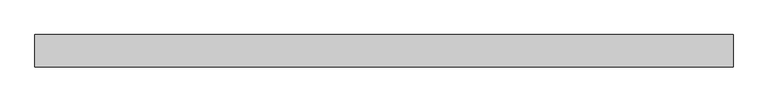
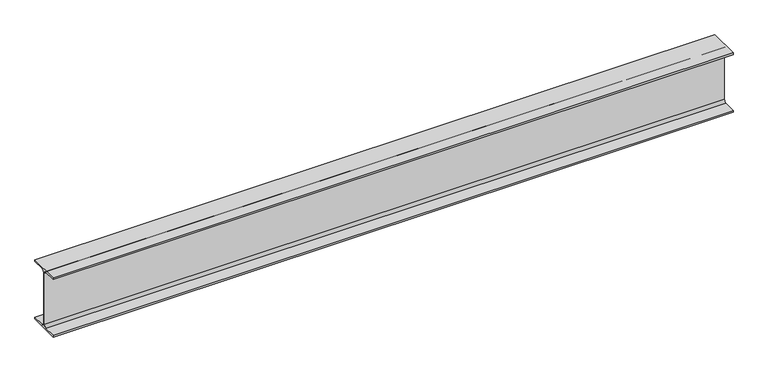
"""IFC4 building model written with IfcOpenShell, lengths in millimetres: beam geometry, Steel Framing_H_KS : H_SB_AR_S02_H-300x150x6.5x9_WG1."""

from ifc_helpers import new_model, si_unit, point, frame, frame_2d, origin, place, context, project, spatial, polyline, circle_curve, trimmed, segment, composite_curve, outline, extrude, source, transform, mapped, element, save


def beam_50cceba7(model_context):
    return source(origin(), model_context, "Body", "SweptSolid", [
        extrude(outline(composite_curve([segment(polyline([(75.0, -141.0), (75.0, -150.0), (-75.0, -150.0), (-75.0, -141.0), (-16.25, -141.0)]), True, "CONTINUOUS"), segment(trimmed(circle_curve(frame_2d((-16.25, -128.0)), 13.0), [point((-16.25, -141.0))], [point((-3.25, -128.0))], True, "CARTESIAN"), True, "CONTINUOUS"), segment(polyline([(-3.25, -128.0), (-3.25, 128.0)]), True, "CONTINUOUS"), segment(trimmed(circle_curve(frame_2d((-16.25, 128.0)), 13.0), [point((-3.25, 128.0))], [point((-16.25, 141.0))], True, "CARTESIAN"), True, "CONTINUOUS"), segment(polyline([(-16.25, 141.0), (-75.0, 141.0), (-75.0, 150.0), (75.0, 150.0), (75.0, 141.0), (16.25, 141.0)]), True, "CONTINUOUS"), segment(trimmed(circle_curve(frame_2d((16.25, 128.0)), 13.0), [point((16.25, 141.0))], [point((3.25, 128.0))], True, "CARTESIAN"), True, "CONTINUOUS"), segment(polyline([(3.25, 128.0), (3.25, -128.0)]), True, "CONTINUOUS"), segment(trimmed(circle_curve(frame_2d((16.25, -128.0)), 13.0), [point((3.25, -128.0))], [point((16.25, -141.0))], True, "CARTESIAN"), True, "CONTINUOUS"), segment(polyline([(16.25, -141.0), (75.0, -141.0)]), True, "CONTINUOUS")], self_intersect=False)), frame((-1587.3, 0.0, 0.0), z_axis=(1.0, 0.0, 0.0), x_axis=(0.0, 1.0, 0.0)), (0.0, 0.0, 1.0), 3249.6),
    ])


if __name__ == "__main__":
    model = new_model("IFC4")
    model_context = context("Model", 3, world=origin())
    ifc_project = project(units=[si_unit("LENGTHUNIT", "METRE", prefix="MILLI")], contexts=[model_context])
    site = spatial("IfcSite", under=ifc_project)
    building = spatial("IfcBuilding", under=site)
    placement = place(None, origin())
    beam_shape = beam_50cceba7(model_context)
    element("IfcBeam", 1, ObjectType="Steel Framing_H_KS : H_SB_AR_S02_H-300x150x6.5x9_WG1", at=placement, inside=building, context=model_context, shape_type="MappedRepresentation", body=[
        mapped(beam_shape, transform((0.0, 0.0, 0.0), x_axis=(1.0, 0.0, 0.0), y_axis=(0.0, 1.0, 0.0), z_axis=(0.0, 0.0, 1.0))),
    ])
    save(model, "model.ifc")

# Revit data of these elements
# Type "Steel Framing_H_KS : H_SB_AR_S02_H-300x150x6.5x9_WG1"
#   Type Comments = "MAIN"
#   Type Mark = "WG1"
#   H_SectionID = "H-300x150x6.5x9"
#   H_Ratio for Additional Steel Plate = 0.2
#   Width = 15.0 cm
#   Web Thickness = 0.65 cm
#   Web Fillet = 1.3 cm
#   Warping Constant = 107000.0 cm⁶
#   Torsional Moment of Inertia = 9.9539 cm⁴
#   Section Area = 46.78 cm²
#   Plastic Modulus weak axis = 105.0 cm³
#   Plastic Modulus strong axis = 542.0 cm³
#   Perimeter = 1.17 m²/m
#   Nominal Weight = 36.70 kgf/m
#   Moment of Inertia weak axis = 508.00 cm⁴
#   Moment of Inertia strong axis = 7210.00 cm⁴
#   Height = 30.0 cm
#   Flange Thickness = 0.9 cm
#   Elastic Modulus weak axis = 67.7 cm³
#   Elastic Modulus strong axis = 481.0 cm³
#   Centroid Vertical = 15.0 cm
#   Centroid Horizontal = 7.5 cm
#   Bolt Spacing = 8.89 cm
#   Length [instance default] = 1500 mm
#   Structural Material [instance default] = Steel, 45-345
#   Section Name Key = ""
#   Assembly Code = ""
# Element 1 (IfcBeam, "Steel Framing_H_KS : H_SB_AR_S02_H-300x150x6.5x9_WG1")
#   Materials on its faces: "Steel, 45-345"
# Materials
#   "Steel, 45-345": class "Metal", colour RGB 189 187 185, transparency 0, Description = "Steel 345 MPa", Cost = 0
